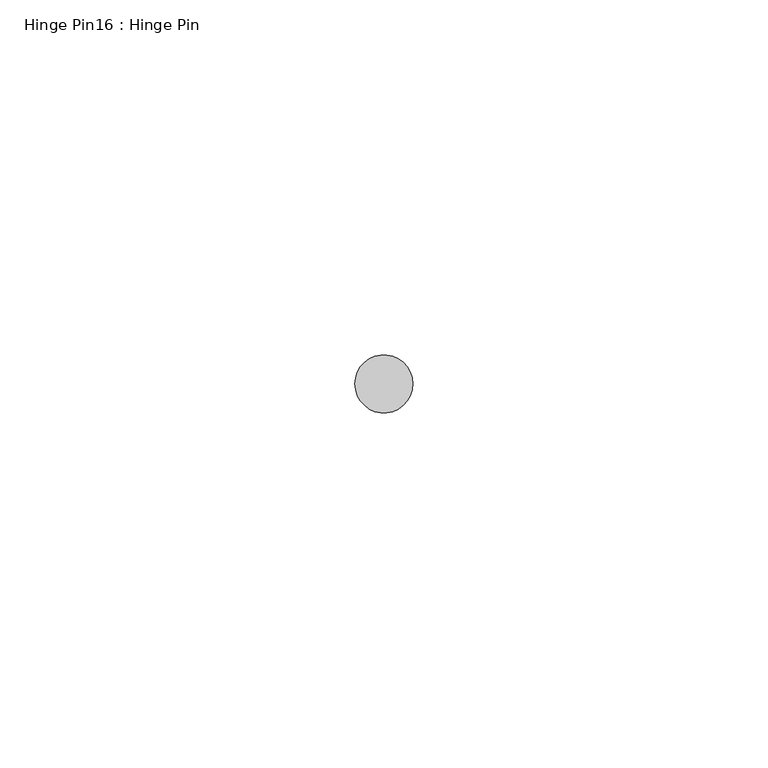
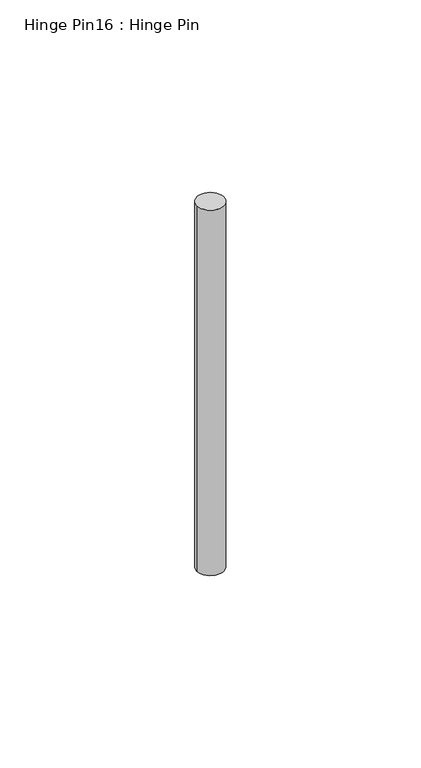
"""IFC4 building model written with IfcOpenShell, lengths in millimetres: proxy geometry, Hinge Pin16 : Hinge Pin."""

import ifcopenshell
import ifcopenshell.guid

model = None  # the IFC model being written
_history = None  # IfcOwnerHistory: only IFC2X3 demands one
_inside = {}  # id of a spatial element -> (the spatial element, [elements in it])
_under = {}  # id of a project, library or spatial element -> (it, [spatial elements below it])
_declared = {}  # id of a project -> (the project, [libraries it declares])
_typed = {}  # id of a type object -> (the type object, [elements of that type])
_made_of = {}  # id of a material, layer set ... -> (it, [elements and type objects made of it])


def new_model(schema):
    """Start an empty IFC model of exactly this schema.

    Asked for "IFC4X3", IfcOpenShell would pick the latest addendum, in which some entities
    have other attributes; the version numbers below select the first issue.
    IFC2X3 requires an IfcOwnerHistory on every rooted entity: one is made here for all.
    """
    global model, _history
    if schema == "IFC4X3":
        model = ifcopenshell.file(schema_version=(4, 3, 0, 0))
    else:
        model = ifcopenshell.file(schema=schema)
    _inside.clear()
    _under.clear()
    _declared.clear()
    _typed.clear()
    _made_of.clear()
    _history = None
    if model.schema == "IFC2X3":
        org = make("IfcOrganization", Name="unknown")
        user = make(
            "IfcPersonAndOrganization",
            ThePerson=make("IfcPerson", FamilyName="unknown"),
            TheOrganization=org,
        )
        app = make(
            "IfcApplication",
            ApplicationDeveloper=org,
            Version="unknown",
            ApplicationFullName="unknown",
            ApplicationIdentifier="unknown",
        )
        _history = make(
            "IfcOwnerHistory",
            OwningUser=user,
            OwningApplication=app,
            ChangeAction="ADDED",
            CreationDate=0,
        )
    return model


def make(cls, **values):
    """One entity of the class cls with the attributes given. An attribute that is None is left unset."""
    return model.create_entity(
        cls, **{name: value for name, value in values.items() if value is not None}
    )


def rooted(cls, **values):
    """An entity with a GlobalId (a new one), such as an element, a storey or a relation."""
    return make(cls, GlobalId=ifcopenshell.guid.new(), OwnerHistory=_history, **values)


def si_unit(unit_type, name, prefix=None):
    """IfcSIUnit, for example si_unit("LENGTHUNIT", "METRE", prefix="MILLI")."""
    return make("IfcSIUnit", UnitType=unit_type, Prefix=prefix, Name=name)


def assignment(units):
    """IfcUnitAssignment: the units of a project."""
    return None if units is None else make("IfcUnitAssignment", Units=units)


def point(xyz):
    """IfcCartesianPoint."""
    return None if xyz is None else make("IfcCartesianPoint", Coordinates=xyz)


def direction(xyz):
    """IfcDirection."""
    return None if xyz is None else make("IfcDirection", DirectionRatios=xyz)


def frame(location, z_axis=None, x_axis=None):
    """IfcAxis2Placement3D, a coordinate frame: its origin and axes. An axis left out is left unset."""
    return make(
        "IfcAxis2Placement3D",
        Location=point(location),
        Axis=direction(z_axis),
        RefDirection=direction(x_axis),
    )


def frame_2d(location, x_axis=None):
    """IfcAxis2Placement2D, a coordinate frame in the plane: its origin and x axis."""
    return make(
        "IfcAxis2Placement2D", Location=point(location), RefDirection=direction(x_axis)
    )


def origin():
    """The frame at (0, 0, 0) with its axes left unset."""
    return frame((0.0, 0.0, 0.0))


def place(relative_to, where):
    """IfcLocalPlacement: puts the frame where relative to a parent placement (None: the world)."""
    return make(
        "IfcLocalPlacement", PlacementRelTo=relative_to, RelativePlacement=where
    )


def context(
    kind, dimensions, precision=None, world=None, true_north=None, identifier=None
):
    """IfcGeometricRepresentationContext, for example the 3D "Model" context."""
    return make(
        "IfcGeometricRepresentationContext",
        ContextIdentifier=identifier,
        ContextType=kind,
        CoordinateSpaceDimension=dimensions,
        Precision=precision,
        WorldCoordinateSystem=world,
        TrueNorth=true_north,
    )


def project(units=None, contexts=None):
    """IfcProject with its units and contexts."""
    return rooted(
        "IfcProject",
        Name="project",
        RepresentationContexts=contexts,
        UnitsInContext=assignment(units),
    )


def spatial(cls, under=None, at=None, **own):
    """A site, building, storey or space (cls), placed at a placement, below another one or the project."""
    s = rooted(cls, ObjectPlacement=at, **own)
    if under is not None:
        _under.setdefault(under.id(), (under, []))[1].append(s)
    return s


def circle_curve(where, radius):
    """IfcCircle in the frame where."""
    return make("IfcCircle", Position=where, Radius=radius)


def trimmed(basis, trim1, trim2, sense, master):
    """IfcTrimmedCurve: the piece of a basis curve between two trims."""
    return make(
        "IfcTrimmedCurve",
        BasisCurve=basis,
        Trim1=trim1,
        Trim2=trim2,
        SenseAgreement=sense,
        MasterRepresentation=master,
    )


def segment(curve, same_sense, transition):
    """IfcCompositeCurveSegment."""
    return make(
        "IfcCompositeCurveSegment",
        Transition=transition,
        SameSense=same_sense,
        ParentCurve=curve,
    )


def composite_curve(segments, self_intersect=None):
    """IfcCompositeCurve: segments joined end to end."""
    return make("IfcCompositeCurve", Segments=segments, SelfIntersect=self_intersect)


def outline(outer, holes=None, kind="AREA"):
    """IfcArbitraryClosedProfileDef: a profile drawn as a closed curve; with holes, ...WithVoids."""
    if holes is None:
        return make("IfcArbitraryClosedProfileDef", ProfileType=kind, OuterCurve=outer)
    return make(
        "IfcArbitraryProfileDefWithVoids",
        ProfileType=kind,
        OuterCurve=outer,
        InnerCurves=holes,
    )


def extrude(swept, where, along, depth):
    """IfcExtrudedAreaSolid: the profile swept, set in the frame where, extruded along a direction by depth."""
    return make(
        "IfcExtrudedAreaSolid",
        SweptArea=swept,
        Position=where,
        ExtrudedDirection=direction(along),
        Depth=depth,
    )


def shape(context_of_items, identifier, shape_type, items):
    """IfcShapeRepresentation: the items that make up one representation, for example the "Body"."""
    return make(
        "IfcShapeRepresentation",
        ContextOfItems=context_of_items,
        RepresentationIdentifier=identifier,
        RepresentationType=shape_type,
        Items=items,
    )


def source(mapping_origin, context_of_items, identifier, shape_type, items):
    """IfcRepresentationMap: a shape defined once, which mapped items show again and again."""
    return make(
        "IfcRepresentationMap",
        MappingOrigin=mapping_origin,
        MappedRepresentation=shape(context_of_items, identifier, shape_type, items),
    )


def transform(
    local_origin,
    x_axis=None,
    y_axis=None,
    z_axis=None,
    scale=None,
    scale2=None,
    scale3=None,
    uniform=True,
):
    """IfcCartesianTransformationOperator3D, or its non-uniform kind. x_axis, y_axis, z_axis: its Axis1, 2, 3."""
    if uniform:
        return make(
            "IfcCartesianTransformationOperator3D",
            Axis1=direction(x_axis),
            Axis2=direction(y_axis),
            LocalOrigin=point(local_origin),
            Scale=scale,
            Axis3=direction(z_axis),
        )
    return make(
        "IfcCartesianTransformationOperator3DnonUniform",
        Axis1=direction(x_axis),
        Axis2=direction(y_axis),
        LocalOrigin=point(local_origin),
        Scale=scale,
        Axis3=direction(z_axis),
        Scale2=scale2,
        Scale3=scale3,
    )


def mapped(mapping_source, mapping_target):
    """IfcMappedItem: shows the shape of a source again, moved by a transform."""
    return make(
        "IfcMappedItem", MappingSource=mapping_source, MappingTarget=mapping_target
    )


def made_of(thing, what):
    """Note that an element or type object is made of a material, layer set ...; save() writes the relation."""
    if what is not None:
        _made_of.setdefault(what.id(), (what, []))[1].append(thing)
    return thing


def element(
    cls,
    number,
    at=None,
    inside=None,
    cuts=None,
    type_object=None,
    material=None,
    context=None,
    identifier="Body",
    shape_type=None,
    held_by="IfcProductDefinitionShape",
    body=None,
    shapes=None,
    **own,
):
    """One element of the class cls, such as IfcWall. Its Tag is "e" and its number.

    at: its placement. inside: the storey or other place that contains it. cuts: it is an
    opening in that element (IfcRelVoidsElement). A single representation is given by context,
    identifier, shape_type and body (its items); several are given by shapes. held_by: the class
    of the entity that holds the representations. save() writes the other relations.
    """
    e = rooted(cls, Tag="e%d" % number, ObjectPlacement=at, **own)
    if body is not None:
        shapes = [shape(context, identifier, shape_type, body)]
    if shapes is not None:
        e.Representation = make(held_by, Representations=shapes)
    if inside is not None:
        _inside.setdefault(inside.id(), (inside, []))[1].append(e)
    if cuts is not None:
        rooted(
            "IfcRelVoidsElement", RelatingBuildingElement=cuts, RelatedOpeningElement=e
        )
    if type_object is not None:
        _typed.setdefault(type_object.id(), (type_object, []))[1].append(e)
    return made_of(e, material)


def aggregate(whole, parts):
    """IfcRelAggregates: a whole, such as a stair, and the parts it consists of."""
    return rooted("IfcRelAggregates", RelatingObject=whole, RelatedObjects=parts)


def save(model, path):
    """Write the relations noted so far, then the file.

    IfcRelAggregates (storeys below a building ...), IfcRelContainedInSpatialStructure (elements
    in a storey), IfcRelDefinesByType, IfcRelAssociatesMaterial and IfcRelDeclares: one each for
    every whole, place, type object, material and project.
    """
    for whole, parts in _under.values():
        aggregate(whole, parts)
    for where, things in _inside.values():
        rooted(
            "IfcRelContainedInSpatialStructure",
            RelatedElements=things,
            RelatingStructure=where,
        )
    for kind, things in _typed.values():
        rooted("IfcRelDefinesByType", RelatedObjects=things, RelatingType=kind)
    for what, things in _made_of.values():
        rooted("IfcRelAssociatesMaterial", RelatedObjects=things, RelatingMaterial=what)
    for by, libraries in _declared.values():
        rooted("IfcRelDeclares", RelatingContext=by, RelatedDefinitions=libraries)
    model.write(path)


def hinge_pin16_hinge_pin_7876437f(model_context):
    return source(origin(), model_context, "Body", "SweptSolid", [
        extrude(outline(composite_curve([segment(trimmed(circle_curve(frame_2d((587319.1320739, -533984.6777841)), 4.0894), [point((587315.0426739, -533984.6777841))], [point((587323.2214739, -533984.6777841))], False, "CARTESIAN"), True, "CONTINUOUS"), segment(trimmed(circle_curve(frame_2d((587319.1320739, -533984.6777841)), 4.0894), [point((587323.2214739, -533984.6777841))], [point((587315.0426739, -533984.6777841))], False, "CARTESIAN"), True, "CONTINUOUS")], self_intersect=False)), frame((0.0, 0.0, 1941.3140625), z_axis=(0.0, 0.0, 1.0), x_axis=(1.0, 0.0, 0.0)), (0.0, 0.0, 1.0), 117.871875),
    ])


if __name__ == "__main__":
    model = new_model("IFC4")
    model_context = context("Model", 3, world=origin())
    ifc_project = project(units=[si_unit("LENGTHUNIT", "METRE", prefix="MILLI")], contexts=[model_context])
    site = spatial("IfcSite", under=ifc_project)
    building = spatial("IfcBuilding", under=site)
    placement = place(None, origin())
    hinge_pin16_hinge_pin_shape = hinge_pin16_hinge_pin_7876437f(model_context)
    element("IfcBuildingElementProxy", 1, Name="Hinge Pin16 : Hinge Pin", ObjectType="Hinge Pin16 : Hinge Pin", at=placement, inside=building, context=model_context, shape_type="MappedRepresentation", body=[
        mapped(hinge_pin16_hinge_pin_shape, transform((0.0, 0.0, 0.0), x_axis=(1.0, 0.0, 0.0), y_axis=(0.0, 1.0, 0.0), z_axis=(0.0, 0.0, 1.0))),
    ])
    save(model, "model.ifc")

# Revit data of these elements
# Element 1 (IfcBuildingElementProxy, "Hinge Pin16 : Hinge Pin")
#   Materials on its faces: "6\"X6\" WELD-ON STL BUTT HINGE"
# Materials
#   "6\"X6\" WELD-ON STL BUTT HINGE": class "Metal", colour RGB 189 187 185, transparency 0, Description = "Carbon steel", Cost = 0
